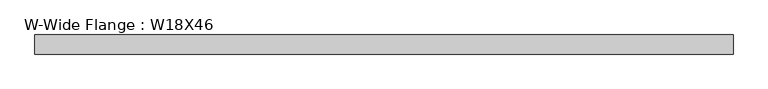
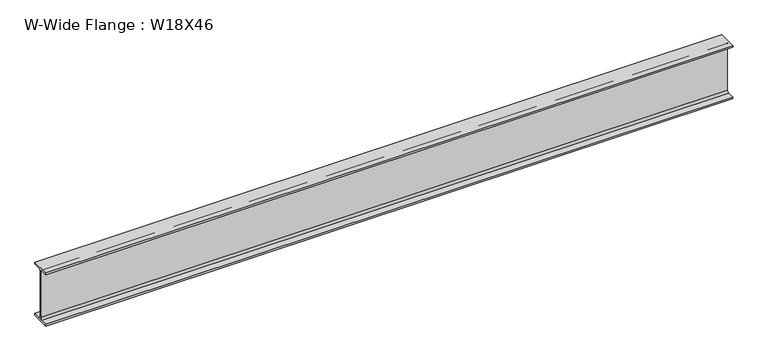
"""IFC4 building model written with IfcOpenShell, lengths in millimetres: beam geometry, W-Wide Flange : W18X46."""

import ifcopenshell
import ifcopenshell.guid

model = None  # the IFC model being written
_history = None  # IfcOwnerHistory: only IFC2X3 demands one
_inside = {}  # id of a spatial element -> (the spatial element, [elements in it])
_under = {}  # id of a project, library or spatial element -> (it, [spatial elements below it])
_declared = {}  # id of a project -> (the project, [libraries it declares])
_typed = {}  # id of a type object -> (the type object, [elements of that type])
_made_of = {}  # id of a material, layer set ... -> (it, [elements and type objects made of it])


def new_model(schema):
    """Start an empty IFC model of exactly this schema.

    Asked for "IFC4X3", IfcOpenShell would pick the latest addendum, in which some entities
    have other attributes; the version numbers below select the first issue.
    IFC2X3 requires an IfcOwnerHistory on every rooted entity: one is made here for all.
    """
    global model, _history
    if schema == "IFC4X3":
        model = ifcopenshell.file(schema_version=(4, 3, 0, 0))
    else:
        model = ifcopenshell.file(schema=schema)
    _inside.clear()
    _under.clear()
    _declared.clear()
    _typed.clear()
    _made_of.clear()
    _history = None
    if model.schema == "IFC2X3":
        org = make("IfcOrganization", Name="unknown")
        user = make(
            "IfcPersonAndOrganization",
            ThePerson=make("IfcPerson", FamilyName="unknown"),
            TheOrganization=org,
        )
        app = make(
            "IfcApplication",
            ApplicationDeveloper=org,
            Version="unknown",
            ApplicationFullName="unknown",
            ApplicationIdentifier="unknown",
        )
        _history = make(
            "IfcOwnerHistory",
            OwningUser=user,
            OwningApplication=app,
            ChangeAction="ADDED",
            CreationDate=0,
        )
    return model


def make(cls, **values):
    """One entity of the class cls with the attributes given. An attribute that is None is left unset."""
    return model.create_entity(
        cls, **{name: value for name, value in values.items() if value is not None}
    )


def rooted(cls, **values):
    """An entity with a GlobalId (a new one), such as an element, a storey or a relation."""
    return make(cls, GlobalId=ifcopenshell.guid.new(), OwnerHistory=_history, **values)


def si_unit(unit_type, name, prefix=None):
    """IfcSIUnit, for example si_unit("LENGTHUNIT", "METRE", prefix="MILLI")."""
    return make("IfcSIUnit", UnitType=unit_type, Prefix=prefix, Name=name)


def assignment(units):
    """IfcUnitAssignment: the units of a project."""
    return None if units is None else make("IfcUnitAssignment", Units=units)


def point(xyz):
    """IfcCartesianPoint."""
    return None if xyz is None else make("IfcCartesianPoint", Coordinates=xyz)


def direction(xyz):
    """IfcDirection."""
    return None if xyz is None else make("IfcDirection", DirectionRatios=xyz)


def frame(location, z_axis=None, x_axis=None):
    """IfcAxis2Placement3D, a coordinate frame: its origin and axes. An axis left out is left unset."""
    return make(
        "IfcAxis2Placement3D",
        Location=point(location),
        Axis=direction(z_axis),
        RefDirection=direction(x_axis),
    )


def frame_2d(location, x_axis=None):
    """IfcAxis2Placement2D, a coordinate frame in the plane: its origin and x axis."""
    return make(
        "IfcAxis2Placement2D", Location=point(location), RefDirection=direction(x_axis)
    )


def origin():
    """The frame at (0, 0, 0) with its axes left unset."""
    return frame((0.0, 0.0, 0.0))


def place(relative_to, where):
    """IfcLocalPlacement: puts the frame where relative to a parent placement (None: the world)."""
    return make(
        "IfcLocalPlacement", PlacementRelTo=relative_to, RelativePlacement=where
    )


def context(
    kind, dimensions, precision=None, world=None, true_north=None, identifier=None
):
    """IfcGeometricRepresentationContext, for example the 3D "Model" context."""
    return make(
        "IfcGeometricRepresentationContext",
        ContextIdentifier=identifier,
        ContextType=kind,
        CoordinateSpaceDimension=dimensions,
        Precision=precision,
        WorldCoordinateSystem=world,
        TrueNorth=true_north,
    )


def project(units=None, contexts=None):
    """IfcProject with its units and contexts."""
    return rooted(
        "IfcProject",
        Name="project",
        RepresentationContexts=contexts,
        UnitsInContext=assignment(units),
    )


def spatial(cls, under=None, at=None, **own):
    """A site, building, storey or space (cls), placed at a placement, below another one or the project."""
    s = rooted(cls, ObjectPlacement=at, **own)
    if under is not None:
        _under.setdefault(under.id(), (under, []))[1].append(s)
    return s


def polyline(points):
    """IfcPolyline through the points."""
    return make("IfcPolyline", Points=[point(p) for p in points])


def circle_curve(where, radius):
    """IfcCircle in the frame where."""
    return make("IfcCircle", Position=where, Radius=radius)


def trimmed(basis, trim1, trim2, sense, master):
    """IfcTrimmedCurve: the piece of a basis curve between two trims."""
    return make(
        "IfcTrimmedCurve",
        BasisCurve=basis,
        Trim1=trim1,
        Trim2=trim2,
        SenseAgreement=sense,
        MasterRepresentation=master,
    )


def segment(curve, same_sense, transition):
    """IfcCompositeCurveSegment."""
    return make(
        "IfcCompositeCurveSegment",
        Transition=transition,
        SameSense=same_sense,
        ParentCurve=curve,
    )


def composite_curve(segments, self_intersect=None):
    """IfcCompositeCurve: segments joined end to end."""
    return make("IfcCompositeCurve", Segments=segments, SelfIntersect=self_intersect)


def outline(outer, holes=None, kind="AREA"):
    """IfcArbitraryClosedProfileDef: a profile drawn as a closed curve; with holes, ...WithVoids."""
    if holes is None:
        return make("IfcArbitraryClosedProfileDef", ProfileType=kind, OuterCurve=outer)
    return make(
        "IfcArbitraryProfileDefWithVoids",
        ProfileType=kind,
        OuterCurve=outer,
        InnerCurves=holes,
    )


def extrude(swept, where, along, depth):
    """IfcExtrudedAreaSolid: the profile swept, set in the frame where, extruded along a direction by depth."""
    return make(
        "IfcExtrudedAreaSolid",
        SweptArea=swept,
        Position=where,
        ExtrudedDirection=direction(along),
        Depth=depth,
    )


def shape(context_of_items, identifier, shape_type, items):
    """IfcShapeRepresentation: the items that make up one representation, for example the "Body"."""
    return make(
        "IfcShapeRepresentation",
        ContextOfItems=context_of_items,
        RepresentationIdentifier=identifier,
        RepresentationType=shape_type,
        Items=items,
    )


def source(mapping_origin, context_of_items, identifier, shape_type, items):
    """IfcRepresentationMap: a shape defined once, which mapped items show again and again."""
    return make(
        "IfcRepresentationMap",
        MappingOrigin=mapping_origin,
        MappedRepresentation=shape(context_of_items, identifier, shape_type, items),
    )


def transform(
    local_origin,
    x_axis=None,
    y_axis=None,
    z_axis=None,
    scale=None,
    scale2=None,
    scale3=None,
    uniform=True,
):
    """IfcCartesianTransformationOperator3D, or its non-uniform kind. x_axis, y_axis, z_axis: its Axis1, 2, 3."""
    if uniform:
        return make(
            "IfcCartesianTransformationOperator3D",
            Axis1=direction(x_axis),
            Axis2=direction(y_axis),
            LocalOrigin=point(local_origin),
            Scale=scale,
            Axis3=direction(z_axis),
        )
    return make(
        "IfcCartesianTransformationOperator3DnonUniform",
        Axis1=direction(x_axis),
        Axis2=direction(y_axis),
        LocalOrigin=point(local_origin),
        Scale=scale,
        Axis3=direction(z_axis),
        Scale2=scale2,
        Scale3=scale3,
    )


def mapped(mapping_source, mapping_target):
    """IfcMappedItem: shows the shape of a source again, moved by a transform."""
    return make(
        "IfcMappedItem", MappingSource=mapping_source, MappingTarget=mapping_target
    )


def made_of(thing, what):
    """Note that an element or type object is made of a material, layer set ...; save() writes the relation."""
    if what is not None:
        _made_of.setdefault(what.id(), (what, []))[1].append(thing)
    return thing


def element(
    cls,
    number,
    at=None,
    inside=None,
    cuts=None,
    type_object=None,
    material=None,
    context=None,
    identifier="Body",
    shape_type=None,
    held_by="IfcProductDefinitionShape",
    body=None,
    shapes=None,
    **own,
):
    """One element of the class cls, such as IfcWall. Its Tag is "e" and its number.

    at: its placement. inside: the storey or other place that contains it. cuts: it is an
    opening in that element (IfcRelVoidsElement). A single representation is given by context,
    identifier, shape_type and body (its items); several are given by shapes. held_by: the class
    of the entity that holds the representations. save() writes the other relations.
    """
    e = rooted(cls, Tag="e%d" % number, ObjectPlacement=at, **own)
    if body is not None:
        shapes = [shape(context, identifier, shape_type, body)]
    if shapes is not None:
        e.Representation = make(held_by, Representations=shapes)
    if inside is not None:
        _inside.setdefault(inside.id(), (inside, []))[1].append(e)
    if cuts is not None:
        rooted(
            "IfcRelVoidsElement", RelatingBuildingElement=cuts, RelatedOpeningElement=e
        )
    if type_object is not None:
        _typed.setdefault(type_object.id(), (type_object, []))[1].append(e)
    return made_of(e, material)


def aggregate(whole, parts):
    """IfcRelAggregates: a whole, such as a stair, and the parts it consists of."""
    return rooted("IfcRelAggregates", RelatingObject=whole, RelatedObjects=parts)


def save(model, path):
    """Write the relations noted so far, then the file.

    IfcRelAggregates (storeys below a building ...), IfcRelContainedInSpatialStructure (elements
    in a storey), IfcRelDefinesByType, IfcRelAssociatesMaterial and IfcRelDeclares: one each for
    every whole, place, type object, material and project.
    """
    for whole, parts in _under.values():
        aggregate(whole, parts)
    for where, things in _inside.values():
        rooted(
            "IfcRelContainedInSpatialStructure",
            RelatedElements=things,
            RelatingStructure=where,
        )
    for kind, things in _typed.values():
        rooted("IfcRelDefinesByType", RelatedObjects=things, RelatingType=kind)
    for what, things in _made_of.values():
        rooted("IfcRelAssociatesMaterial", RelatedObjects=things, RelatingMaterial=what)
    for by, libraries in _declared.values():
        rooted("IfcRelDeclares", RelatingContext=by, RelatedDefinitions=libraries)
    model.write(path)


def w_wide_flange_w18x46_a2dbce11(model_context):
    return source(origin(), model_context, "Body", "SweptSolid", [
        extrude(outline(composite_curve([segment(polyline([(76.962, -214.503), (76.962, -229.87), (-76.962, -229.87), (-76.962, -214.503), (-20.955, -214.503)]), True, "CONTINUOUS"), segment(trimmed(circle_curve(frame_2d((-20.955, -198.12)), 16.383), [point((-20.955, -214.503))], [point((-4.572, -198.12))], True, "CARTESIAN"), True, "CONTINUOUS"), segment(polyline([(-4.572, -198.12), (-4.572, 198.12)]), True, "CONTINUOUS"), segment(trimmed(circle_curve(frame_2d((-20.955, 198.12)), 16.383), [point((-4.572, 198.12))], [point((-20.955, 214.503))], True, "CARTESIAN"), True, "CONTINUOUS"), segment(polyline([(-20.955, 214.503), (-76.962, 214.503), (-76.962, 229.87), (76.962, 229.87), (76.962, 214.503), (20.955, 214.503)]), True, "CONTINUOUS"), segment(trimmed(circle_curve(frame_2d((20.955, 198.12)), 16.383), [point((20.955, 214.503))], [point((4.572, 198.12))], True, "CARTESIAN"), True, "CONTINUOUS"), segment(polyline([(4.572, 198.12), (4.572, -198.12)]), True, "CONTINUOUS"), segment(trimmed(circle_curve(frame_2d((20.955, -198.12)), 16.383), [point((4.572, -198.12))], [point((20.955, -214.503))], True, "CARTESIAN"), True, "CONTINUOUS"), segment(polyline([(20.955, -214.503), (76.962, -214.503)]), True, "CONTINUOUS")], self_intersect=False)), frame((-2806.7, 0.0, 0.0), z_axis=(1.0, 0.0, 0.0), x_axis=(0.0, 1.0, 0.0)), (0.0, 0.0, 1.0), 5613.4),
    ])


if __name__ == "__main__":
    model = new_model("IFC4")
    model_context = context("Model", 3, world=origin())
    ifc_project = project(units=[si_unit("LENGTHUNIT", "METRE", prefix="MILLI")], contexts=[model_context])
    site = spatial("IfcSite", under=ifc_project)
    building = spatial("IfcBuilding", under=site)
    placement = place(None, origin())
    w_wide_flange_w18x46_shape = w_wide_flange_w18x46_a2dbce11(model_context)
    element("IfcBeam", 1, ObjectType="W-Wide Flange : W18X46", at=placement, inside=building, context=model_context, shape_type="MappedRepresentation", body=[
        mapped(w_wide_flange_w18x46_shape, transform((0.0, 0.0, 0.0), x_axis=(1.0, 0.0, 0.0), y_axis=(0.0, 1.0, 0.0), z_axis=(0.0, 0.0, 1.0))),
    ])
    save(model, "model.ifc")

# Revit data of these elements
# Type "W-Wide Flange : W18X46"
#   Assembly Code = "B10"
#   W = 46
#   Length [instance default] = 5' - 0"
#   bf = 0' - 6.06"
#   d = 1' - 6.1"
#   k = 0' - 1 1/4"
#   k2 = 0' - 0.645"
#   tf = 0' - 0.605"
#   tw = 0' - 0.36"
#   A = 0.09375 SF
#   Structural Material [instance default] = Steel ASTM A992
# Element 1 (IfcBeam, "W-Wide Flange : W18X46")
#   Materials on its faces: "Steel ASTM A992"
# Materials
#   "Steel ASTM A992": class "Metal", colour RGB 199 199 199, transparency 0, Description = "Structural steel 50ksi", Cost = 0
